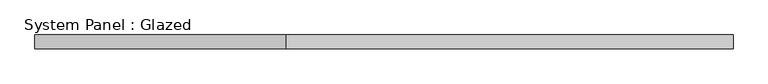
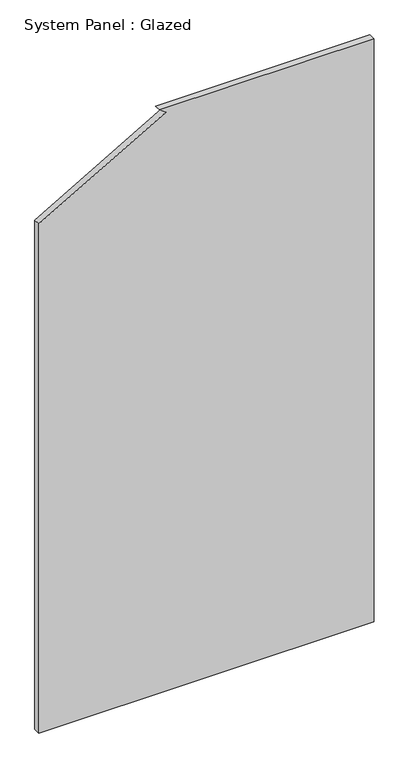
"""IFC4 building model written with IfcOpenShell, lengths in millimetres: plate geometry, System Panel : Glazed."""

from ifc_helpers import new_model, si_unit, frame, origin, place, context, project, spatial, polyline, outline, extrude, source, transform, mapped, element, save


def system_panel_glazed_fe074b21(model_context):
    return source(origin(), model_context, "Body", "SweptSolid", [
        extrude(outline(polyline([(0.0, -639.2857142), (0.0, 639.2857142), (2350.0, 639.2857142), (2350.0, -178.8659873), (2331.6987298, -153.8659873), (2051.4415198, -639.2857142), (0.0, -639.2857142)])), frame((0.0, 24.5, 0.0), z_axis=(0.0, 1.0, 0.0), x_axis=(0.0, 0.0, 1.0)), (0.0, 0.0, 1.0), 25.0),
    ])


if __name__ == "__main__":
    model = new_model("IFC4")
    model_context = context("Model", 3, world=origin())
    ifc_project = project(units=[si_unit("LENGTHUNIT", "METRE", prefix="MILLI")], contexts=[model_context])
    site = spatial("IfcSite", under=ifc_project)
    building = spatial("IfcBuilding", under=site)
    placement = place(None, origin())
    system_panel_glazed_shape = system_panel_glazed_fe074b21(model_context)
    element("IfcPlate", 1, ObjectType="System Panel : Glazed", at=placement, inside=building, context=model_context, shape_type="MappedRepresentation", body=[
        mapped(system_panel_glazed_shape, transform((0.0, 0.0, 0.0), x_axis=(1.0, 0.0, 0.0), y_axis=(0.0, 1.0, 0.0), z_axis=(0.0, 0.0, 1.0))),
    ])
    save(model, "model.ifc")

# Revit data of these elements
# Type "System Panel : Glazed"
#   Construction Type Id = "GSP4R"
#   Analytic Construction = "1/8 in Pilkington single glazing"
#   Visual Light Transmittance = 0.9
#   Solar Heat Gain Coefficient = 0.86
#   Heat Transfer Coefficient (U) = 6.7069 W/(m²·K)
#   Define Thermal Properties by = 1
# Element 1 (IfcPlate, "System Panel : Glazed")
#   Materials on its faces: "Glass"
# Materials
#   "Glass": class "Glass", colour RGB 0 128 192, transparency 0.75, Description = "Soda Lime Glass", Cost = 0
